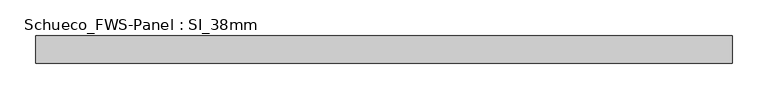
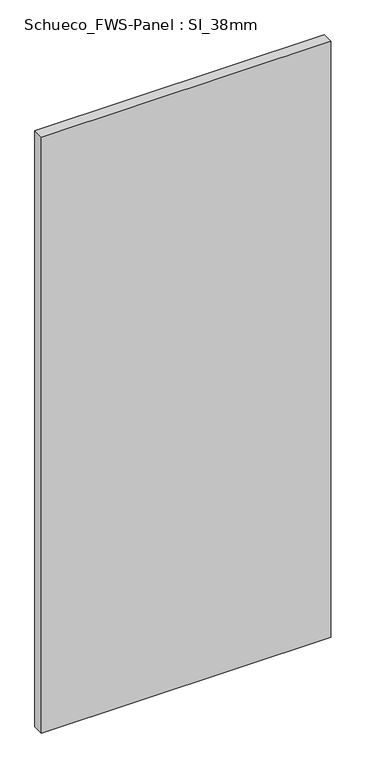
"""IFC4 building model written with IfcOpenShell, lengths in millimetres: plate geometry, Schueco_FWS-Panel : SI_38mm."""

from ifc_helpers import new_model, si_unit, origin, origin_with_axes, place, context, project, spatial, polyline, outline, extrude, source, transform, mapped, element, save


def schueco_fws_panel_si_38mm_3dca22e8(model_context):
    return source(origin(), model_context, "Body", "SweptSolid", [
        extrude(outline(polyline([(-484.0, 0.0), (484.0, 0.0), (484.0, -38.0), (-484.0, -38.0), (-484.0, 0.0)])), origin_with_axes(), (0.0, 0.0, 1.0), 2108.0),
    ])


if __name__ == "__main__":
    model = new_model("IFC4")
    model_context = context("Model", 3, world=origin())
    ifc_project = project(units=[si_unit("LENGTHUNIT", "METRE", prefix="MILLI")], contexts=[model_context])
    site = spatial("IfcSite", under=ifc_project)
    building = spatial("IfcBuilding", under=site)
    placement = place(None, origin())
    schueco_fws_panel_si_38mm_shape = schueco_fws_panel_si_38mm_3dca22e8(model_context)
    element("IfcPlate", 1, ObjectType="Schueco_FWS-Panel : SI_38mm", at=placement, inside=building, context=model_context, shape_type="MappedRepresentation", body=[
        mapped(schueco_fws_panel_si_38mm_shape, transform((0.0, 0.0, 0.0), x_axis=(1.0, 0.0, 0.0), y_axis=(0.0, 1.0, 0.0), z_axis=(0.0, 0.0, 1.0))),
    ])
    save(model, "model.ifc")

# Revit data of these elements
# Type "Schueco_FWS-Panel : SI_38mm"
#   Model = "Panel 38mm"
#   Manufacturer = "Schueco International KG"
#   Analytic Construction = "<Keine Auswahl>"
#   Panel thickness = 38 mm
#   Angle right [instance default] = 0.00°
#   Angle left [instance default] = 0.00°
#   AR [instance default] = 0.00°
#   AL [instance default] = 0.00°
#   FWS SI insert unit = yes
#   FWS HI insert unit = no
#   Det_R [instance default] = yes
#   Det_L [instance default] = yes
#   Panel = Alu
# Element 1 (IfcPlate, "Schueco_FWS-Panel : SI_38mm")
#   Materials on its faces: "Alu"
# Materials
#   "Alu": class "Glas", colour RGB 140 140 140, transparency 0
